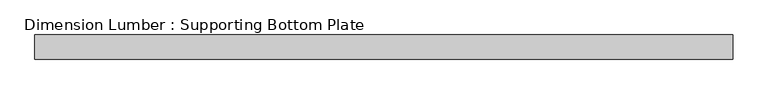
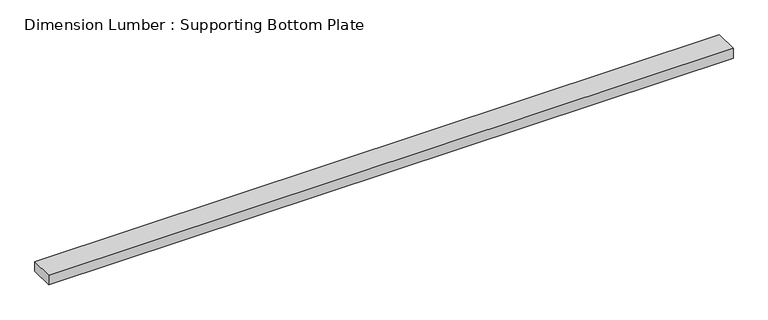
"""IFC4 building model written with IfcOpenShell, lengths in millimetres: beam geometry, Dimension Lumber : Supporting Bottom Plate."""

from ifc_helpers import new_model, si_unit, frame, origin, place, context, project, spatial, polyline, outline, extrude, source, transform, mapped, element, save


def dimension_lumber_supporting_bottom_plate_c90501c4(model_context):
    return source(origin(), model_context, "Body", "SweptSolid", [
        extrude(outline(polyline([(1306.3140625, 44.45), (1306.3140625, -44.45), (-1261.8640625, -44.45), (-1261.8640625, 44.45), (1306.3140625, 44.45)])), frame((0.0, 0.0, -19.05), z_axis=(0.0, 0.0, 1.0), x_axis=(1.0, 0.0, 0.0)), (0.0, 0.0, 1.0), 38.1),
    ])


if __name__ == "__main__":
    model = new_model("IFC4")
    model_context = context("Model", 3, world=origin())
    ifc_project = project(units=[si_unit("LENGTHUNIT", "METRE", prefix="MILLI")], contexts=[model_context])
    site = spatial("IfcSite", under=ifc_project)
    building = spatial("IfcBuilding", under=site)
    placement = place(None, origin())
    dimension_lumber_supporting_bottom_plate_shape = dimension_lumber_supporting_bottom_plate_c90501c4(model_context)
    element("IfcBeam", 1, ObjectType="Dimension Lumber : Supporting Bottom Plate", at=placement, inside=building, context=model_context, shape_type="MappedRepresentation", body=[
        mapped(dimension_lumber_supporting_bottom_plate_shape, transform((0.0, 0.0, 0.0), x_axis=(1.0, 0.0, 0.0), y_axis=(0.0, 1.0, 0.0), z_axis=(0.0, 0.0, 1.0))),
    ])
    save(model, "model.ifc")

# Revit data of these elements
# Type "Dimension Lumber : Supporting Bottom Plate"
#   Assembly Code = "B10"
#   A = 0.0364583 SF
#   Length [instance default] = 5' - 0"
#   b = 0' - 3 1/2"
#   d = 0' - 1 1/2"
#   Structural Material [instance default] = Softwood, Lumber
# Element 1 (IfcBeam, "Dimension Lumber : Supporting Bottom Plate")
#   Structural Material = Douglas Fir #2
#   Materials on its faces: "Douglas Fir #2"
# Materials
#   "Softwood, Lumber": class "Wood", colour RGB 223 192 134, transparency 0, Description = "Pinus Echinata", Cost = 0
#   "Douglas Fir #2": class "Wood", colour RGB 223 192 134, transparency 0, Description = "Pinus Echinata", Cost = 0
